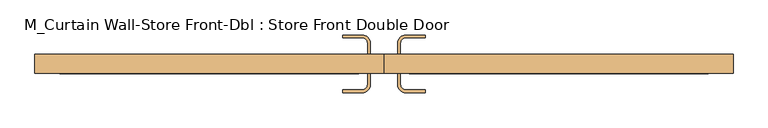
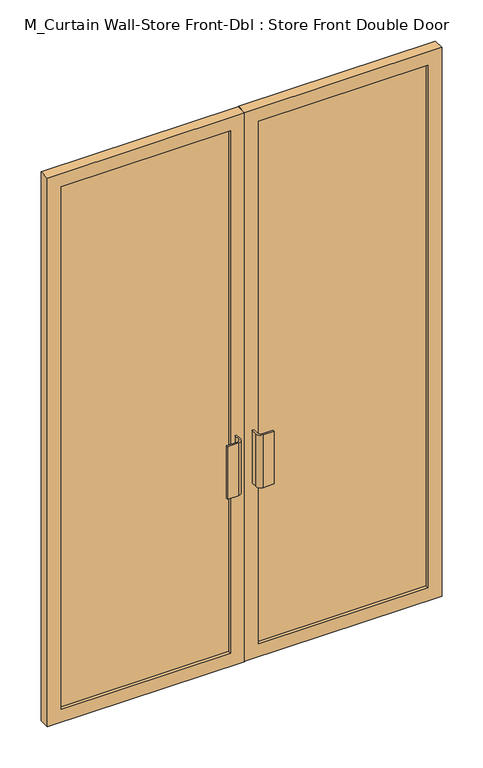
"""IFC4 building model written with IfcOpenShell, lengths in millimetres: door geometry, M_Curtain Wall-Store Front-Dbl : Store Front Double Door."""

from ifc_helpers import new_model, si_unit, point, frame, frame_2d, origin, place, context, project, spatial, polyline, circle_curve, trimmed, segment, composite_curve, outline, extrude, source, transform, mapped, element, save


def m_curtain_wall_store_front_dbl_store_front_double_door_ce2fb254(model_context):
    return source(origin(), model_context, "Body", "SweptSolid", [
        extrude(outline(composite_curve([segment(trimmed(circle_curve(frame_2d((-50.8, -14.85)), 19.05), [point((-31.75, -14.85))], [point((-50.8, -33.9))], False, "CARTESIAN"), True, "CONTINUOUS"), segment(polyline([(-50.8, -33.9), (-95.25, -33.9), (-95.25, -27.55), (-50.8, -27.55)]), True, "CONTINUOUS"), segment(trimmed(circle_curve(frame_2d((-50.8, -14.85)), 12.7), [point((-50.8, -27.55))], [point((-38.1, -14.85))], True, "CARTESIAN"), True, "CONTINUOUS"), segment(polyline([(-38.1, -14.85), (-38.1, 10.55), (-31.75, 10.55), (-31.75, -14.85)]), True, "CONTINUOUS")], self_intersect=False)), frame((0.0, 0.0, 762.0), z_axis=(0.0, 0.0, 1.0), x_axis=(1.0, 0.0, 0.0)), (0.0, 0.0, 1.0), 228.6),
        extrude(outline(composite_curve([segment(polyline([(31.75, -14.85), (31.75, 10.55), (38.1, 10.55), (38.1, -14.85)]), True, "CONTINUOUS"), segment(trimmed(circle_curve(frame_2d((50.8, -14.85)), 12.7), [point((38.1, -14.85))], [point((50.8, -27.55))], True, "CARTESIAN"), True, "CONTINUOUS"), segment(polyline([(50.8, -27.55), (95.25, -27.55), (95.25, -33.9), (50.8, -33.9)]), True, "CONTINUOUS"), segment(trimmed(circle_curve(frame_2d((50.8, -14.85)), 19.05), [point((50.8, -33.9))], [point((31.75, -14.85))], False, "CARTESIAN"), True, "CONTINUOUS")], self_intersect=False)), frame((0.0, 0.0, 762.0), z_axis=(0.0, 0.0, 1.0), x_axis=(1.0, 0.0, 0.0)), (0.0, 0.0, 1.0), 228.6),
        extrude(outline(composite_curve([segment(polyline([(-31.75, 80.4), (-31.75, 55.0), (-38.1, 55.0), (-38.1, 80.4)]), True, "CONTINUOUS"), segment(trimmed(circle_curve(frame_2d((-50.8, 80.4)), 12.7), [point((-38.1, 80.4))], [point((-50.8, 93.1))], True, "CARTESIAN"), True, "CONTINUOUS"), segment(polyline([(-50.8, 93.1), (-95.25, 93.1), (-95.25, 99.45), (-50.8, 99.45)]), True, "CONTINUOUS"), segment(trimmed(circle_curve(frame_2d((-50.8, 80.4)), 19.05), [point((-50.8, 99.45))], [point((-31.75, 80.4))], False, "CARTESIAN"), True, "CONTINUOUS")], self_intersect=False)), frame((0.0, 0.0, 762.0), z_axis=(0.0, 0.0, 1.0), x_axis=(1.0, 0.0, 0.0)), (0.0, 0.0, 1.0), 228.6),
        extrude(outline(composite_curve([segment(trimmed(circle_curve(frame_2d((50.8, 80.4)), 19.05), [point((31.75, 80.4))], [point((50.8, 99.45))], False, "CARTESIAN"), True, "CONTINUOUS"), segment(polyline([(50.8, 99.45), (95.25, 99.45), (95.25, 93.1), (50.8, 93.1)]), True, "CONTINUOUS"), segment(trimmed(circle_curve(frame_2d((50.8, 80.4)), 12.7), [point((50.8, 93.1))], [point((38.1, 80.4))], True, "CARTESIAN"), True, "CONTINUOUS"), segment(polyline([(38.1, 80.4), (38.1, 55.0), (31.75, 55.0), (31.75, 80.4)]), True, "CONTINUOUS")], self_intersect=False)), frame((0.0, 0.0, 762.0), z_axis=(0.0, 0.0, 1.0), x_axis=(1.0, 0.0, 0.0)), (0.0, 0.0, 1.0), 228.6),
        extrude(outline(polyline([(750.35, 23.25), (57.94375, 23.25), (57.94375, 42.3), (750.35, 42.3), (750.35, 23.25)])), frame((0.0, 0.0, 57.15), z_axis=(0.0, 0.0, 1.0), x_axis=(1.0, 0.0, 0.0)), (0.0, 0.0, 1.0), 2260.7),
        extrude(outline(polyline([(-57.94375, 23.25), (-750.35, 23.25), (-750.35, 42.3), (-57.94375, 42.3), (-57.94375, 23.25)])), frame((0.0, 0.0, 57.15), z_axis=(0.0, 0.0, 1.0), x_axis=(1.0, 0.0, 0.0)), (0.0, 0.0, 1.0), 2260.7),
        extrude(outline(polyline([(2375.0, 0.79375), (0.0, 0.79375), (0.0, 807.5), (2375.0, 807.5), (2375.0, 0.79375)]), holes=[polyline([(2317.85, 57.94375), (2317.85, 750.35), (57.15, 750.35), (57.15, 57.94375), (2317.85, 57.94375)])]), frame((0.0, 10.55, 0.0), z_axis=(0.0, 1.0, 0.0), x_axis=(0.0, 0.0, 1.0)), (0.0, 0.0, 1.0), 44.45),
        extrude(outline(polyline([(2375.0, -0.79375), (2375.0, -807.5), (0.0, -807.5), (0.0, -0.79375), (2375.0, -0.79375)]), holes=[polyline([(2317.85, -750.35), (2317.85, -57.94375), (57.15, -57.94375), (57.15, -750.35), (2317.85, -750.35)])]), frame((0.0, 10.55, 0.0), z_axis=(0.0, 1.0, 0.0), x_axis=(0.0, 0.0, 1.0)), (0.0, 0.0, 1.0), 44.45),
    ])


if __name__ == "__main__":
    model = new_model("IFC4")
    model_context = context("Model", 3, world=origin())
    ifc_project = project(units=[si_unit("LENGTHUNIT", "METRE", prefix="MILLI")], contexts=[model_context])
    site = spatial("IfcSite", under=ifc_project)
    building = spatial("IfcBuilding", under=site)
    placement = place(None, origin())
    m_curtain_wall_store_front_dbl_store_front_double_door_shape = m_curtain_wall_store_front_dbl_store_front_double_door_ce2fb254(model_context)
    element("IfcDoor", 1, ObjectType="M_Curtain Wall-Store Front-Dbl : Store Front Double Door", at=placement, inside=building, context=model_context, shape_type="MappedRepresentation", body=[
        mapped(m_curtain_wall_store_front_dbl_store_front_double_door_shape, transform((0.0, 0.0, 0.0), x_axis=(1.0, 0.0, 0.0), y_axis=(0.0, 1.0, 0.0), z_axis=(0.0, 0.0, 1.0))),
    ])
    save(model, "model.ifc")

# Revit data of these elements
# Type "M_Curtain Wall-Store Front-Dbl : Store Front Double Door"
#   Type Mark = "33"
#   Offset = 55 mm
#   Function = 1
#   Material = Metal - Aluminum
#   Glazing Material = Glass
#   Assembly Code = ""
# Element 1 (IfcDoor, "M_Curtain Wall-Store Front-Dbl : Store Front Double Door")
#   Materials on its faces: "Metal - Aluminum", "Glass"
# Materials
#   "Metal - Aluminum": class "Metal", colour RGB 247 247 247, transparency 0
#   "Glass": class "Glass", colour RGB 0 128 192, transparency 0.9
